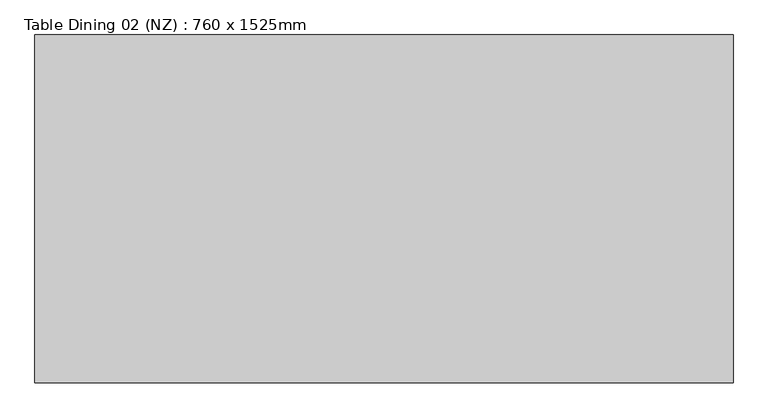
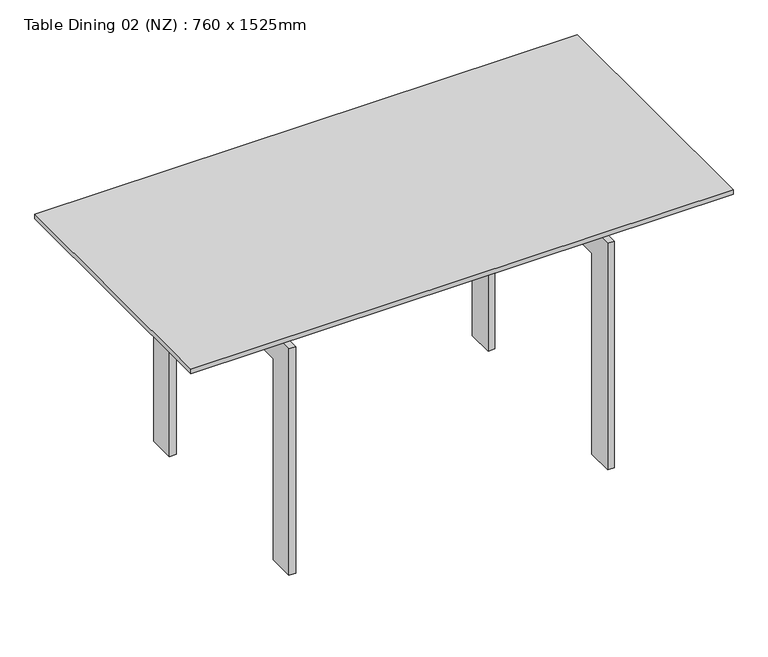
"""IFC4 building model written with IfcOpenShell, lengths in millimetres: furniture geometry, Table Dining 02 (NZ) : 760 x 1525mm."""

from ifc_helpers import new_model, si_unit, frame, origin, place, context, project, spatial, polyline, outline, extrude, source, transform, mapped, element, save


def table_dining_02_nz_760_x_1525mm_768527a3(model_context):
    return source(origin(), model_context, "Body", "SweptSolid", [
        extrude(outline(polyline([(780.7657667, 475.2110778), (780.7657667, -284.7889222), (-744.2342333, -284.7889222), (-744.2342333, 475.2110778), (780.7657667, 475.2110778)])), frame((0.0, 0.0, 737.3), z_axis=(0.0, 0.0, 1.0), x_axis=(1.0, 0.0, 0.0)), (0.0, 0.0, 1.0), 12.7),
        extrude(outline(polyline([(679.1657667, 297.7823857), (679.1657667, 272.3823857), (-642.6342333, 272.3823857), (-642.6342333, 297.7823857), (679.1657667, 297.7823857)])), frame((0.0, 0.0, 673.8), z_axis=(0.0, 0.0, 1.0), x_axis=(1.0, 0.0, 0.0)), (0.0, 0.0, 1.0), 63.5),
        extrude(outline(polyline([(679.1657667, -82.5889222), (679.1657667, -107.9889222), (-642.6342333, -107.9889222), (-642.6342333, -82.5889222), (679.1657667, -82.5889222)])), frame((0.0, 0.0, 673.8), z_axis=(0.0, 0.0, 1.0), x_axis=(1.0, 0.0, 0.0)), (0.0, 0.0, 1.0), 63.5),
        extrude(outline(polyline([(424.4110778, 0.0), (348.2110778, 0.0), (348.2110778, 597.6), (-157.7889222, 597.6), (-157.7889222, 0.0), (-233.9889222, 0.0), (-233.9889222, 673.8), (424.4110778, 673.8), (424.4110778, 0.0)])), frame((456.9157667, 0.0, 0.0), z_axis=(1.0, 0.0, 0.0), x_axis=(0.0, 1.0, 0.0)), (0.0, 0.0, 1.0), 19.05),
        extrude(outline(polyline([(424.4110778, 673.8), (424.4110778, 0.0), (348.2110778, 0.0), (348.2110778, 597.6), (-157.7889222, 597.6), (-157.7889222, 0.0), (-233.9889222, 0.0), (-233.9889222, 673.8), (424.4110778, 673.8)])), frame((-439.4342333, 0.0, 0.0), z_axis=(1.0, 0.0, 0.0), x_axis=(0.0, 1.0, 0.0)), (0.0, 0.0, 1.0), 19.05),
    ])


if __name__ == "__main__":
    model = new_model("IFC4")
    model_context = context("Model", 3, world=origin())
    ifc_project = project(units=[si_unit("LENGTHUNIT", "METRE", prefix="MILLI")], contexts=[model_context])
    site = spatial("IfcSite", under=ifc_project)
    building = spatial("IfcBuilding", under=site)
    placement = place(None, origin())
    table_dining_02_nz_760_x_1525mm_shape = table_dining_02_nz_760_x_1525mm_768527a3(model_context)
    element("IfcFurniture", 1, ObjectType="Table Dining 02 (NZ) : 760 x 1525mm", at=placement, inside=building, context=model_context, shape_type="MappedRepresentation", body=[
        mapped(table_dining_02_nz_760_x_1525mm_shape, transform((0.0, 0.0, 0.0), x_axis=(1.0, 0.0, 0.0), y_axis=(0.0, 1.0, 0.0), z_axis=(0.0, 0.0, 1.0))),
    ])
    save(model, "model.ifc")

# Revit data of these elements
# Type "Table Dining 02 (NZ) : 760 x 1525mm"
#   Height = 750 mm
#   Length = 1525 mm
#   Width = 760 mm
#   Base Material = Metal - Chrome
#   Top Material = Glass - Clear, Grey
#   Assembly Code = ""
# Element 1 (IfcFurniture, "Table Dining 02 (NZ) : 760 x 1525mm")
#   Materials on its faces: "Metal - Chrome", "Glass - Clear, Grey"
# Materials
#   "Metal - Chrome": class "Metal", colour RGB 17 17 17, transparency 0
#   "Glass - Clear, Grey": class "Glass", colour RGB 252 255 255, transparency 0.64
